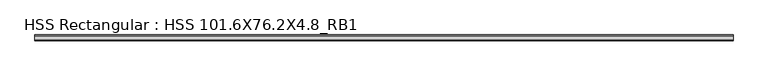
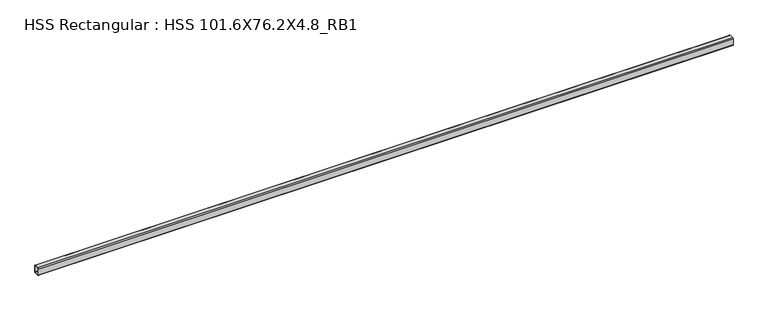
"""IFC4 building model written with IfcOpenShell, lengths in millimetres: beam geometry, HSS Rectangular : HSS 101.6X76.2X4.8_RB1."""

from ifc_helpers import new_model, si_unit, point, frame, frame_2d, origin, place, context, project, spatial, polyline, circle_curve, trimmed, segment, composite_curve, outline, extrude, source, transform, mapped, element, save


def hss_rectangular_hss_101_6x76_2x4_8_rb1_6835c934(model_context):
    return source(origin(), model_context, "Body", "SweptSolid", [
        extrude(outline(composite_curve([segment(trimmed(circle_curve(frame_2d((-28.575, 41.275)), 9.525), [point((-38.1, 41.275))], [point((-28.575, 50.8))], False, "CARTESIAN"), True, "CONTINUOUS"), segment(polyline([(-28.575, 50.8), (28.575, 50.8)]), True, "CONTINUOUS"), segment(trimmed(circle_curve(frame_2d((28.575, 41.275)), 9.525), [point((28.575, 50.8))], [point((38.1, 41.275))], False, "CARTESIAN"), True, "CONTINUOUS"), segment(polyline([(38.1, 41.275), (38.1, -41.275)]), True, "CONTINUOUS"), segment(trimmed(circle_curve(frame_2d((28.575, -41.275)), 9.525), [point((38.1, -41.275))], [point((28.575, -50.8))], False, "CARTESIAN"), True, "CONTINUOUS"), segment(polyline([(28.575, -50.8), (-28.575, -50.8)]), True, "CONTINUOUS"), segment(trimmed(circle_curve(frame_2d((-28.575, -41.275)), 9.525), [point((-28.575, -50.8))], [point((-38.1, -41.275))], False, "CARTESIAN"), True, "CONTINUOUS"), segment(polyline([(-38.1, -41.275), (-38.1, 41.275)]), True, "CONTINUOUS")], self_intersect=False), holes=[composite_curve([segment(polyline([(28.575, 46.0375), (-28.575, 46.0375)]), True, "CONTINUOUS"), segment(trimmed(circle_curve(frame_2d((-28.575, 41.275)), 4.7625), [point((-28.575, 46.0375))], [point((-33.3375, 41.275))], True, "CARTESIAN"), True, "CONTINUOUS"), segment(polyline([(-33.3375, 41.275), (-33.3375, -41.275)]), True, "CONTINUOUS"), segment(trimmed(circle_curve(frame_2d((-28.575, -41.275)), 4.7625), [point((-33.3375, -41.275))], [point((-28.575, -46.0375))], True, "CARTESIAN"), True, "CONTINUOUS"), segment(polyline([(-28.575, -46.0375), (28.575, -46.0375)]), True, "CONTINUOUS"), segment(trimmed(circle_curve(frame_2d((28.575, -41.275)), 4.7625), [point((28.575, -46.0375))], [point((33.3375, -41.275))], True, "CARTESIAN"), True, "CONTINUOUS"), segment(polyline([(33.3375, -41.275), (33.3375, 41.275)]), True, "CONTINUOUS"), segment(trimmed(circle_curve(frame_2d((28.575, 41.275)), 4.7625), [point((33.3375, 41.275))], [point((28.575, 46.0375))], True, "CARTESIAN"), True, "CONTINUOUS")], self_intersect=False)]), frame((-7489.089, 0.0, 0.0), z_axis=(1.0, 0.0, 0.0), x_axis=(0.0, 1.0, 0.0)), (0.0, 0.0, 1.0), 9027.189),
    ])


if __name__ == "__main__":
    model = new_model("IFC4")
    model_context = context("Model", 3, world=origin())
    ifc_project = project(units=[si_unit("LENGTHUNIT", "METRE", prefix="MILLI")], contexts=[model_context])
    site = spatial("IfcSite", under=ifc_project)
    building = spatial("IfcBuilding", under=site)
    placement = place(None, origin())
    hss_rectangular_hss_101_6x76_2x4_8_rb1_shape = hss_rectangular_hss_101_6x76_2x4_8_rb1_6835c934(model_context)
    element("IfcBeam", 1, ObjectType="HSS Rectangular : HSS 101.6X76.2X4.8_RB1", at=placement, inside=building, context=model_context, shape_type="MappedRepresentation", body=[
        mapped(hss_rectangular_hss_101_6x76_2x4_8_rb1_shape, transform((0.0, 0.0, 0.0), x_axis=(1.0, 0.0, 0.0), y_axis=(0.0, 1.0, 0.0), z_axis=(0.0, 0.0, 1.0))),
    ])
    save(model, "model.ifc")

# Revit data of these elements
# Type "HSS Rectangular : HSS 101.6X76.2X4.8_RB1"
#   Section Name Key = "HSS 4X3X3/16"
#   Assembly Code = "B10"
#   Width = 7.62 cm
#   Wall Nominal Thickness = 0.4763 cm
#   Wall Design Thickness = 0.442 cm
#   Torsional Moment of Inertia = 260.561 cm⁴
#   Torsional Modulus = 61.2876 cm³
#   Section Area = 14.4516 cm²
#   Plastic Modulus weak axis = 40.3122 cm³
#   Plastic Modulus strong axis = 49.1612 cm³
#   Perimeter = 0.881482 m²/m
#   Outer Fillet = 0.9525 cm
#   Nominal Weight = 12.1285 kgf/m
#   Moment of Inertia weak axis = 131.529 cm⁴
#   Moment of Inertia strong axis = 205.202 cm⁴
#   Inner Fillet = 0.4763 cm
#   Height = 10.16 cm
#   Elastic Modulus weak axis = 34.4128 cm³
#   Elastic Modulus strong axis = 40.476 cm³
#   Centroid Vertical = 5.08 cm
#   Centroid Horizontal = 3.81 cm
#   Length [instance default] = 1524 mm
#   Structural Material [instance default] = Steel ASTM A500, Grade B, Rectangular and Square
#   Principal Axes Angle = 0
# Element 1 (IfcBeam, "HSS Rectangular : HSS 101.6X76.2X4.8_RB1")
#   Structural Material = Steel ASTM A992
#   Materials on its faces: "Steel ASTM A992"
# Materials
#   "Steel ASTM A500, Grade B, Rectangular and Square": class "Metal", colour RGB 199 199 199, transparency 0, Description = "Carbon steel", Cost = 0
#   "Steel ASTM A992": class "Metal", colour RGB 199 199 199, transparency 0, Description = "Structural steel 50ksi", Cost = 0
